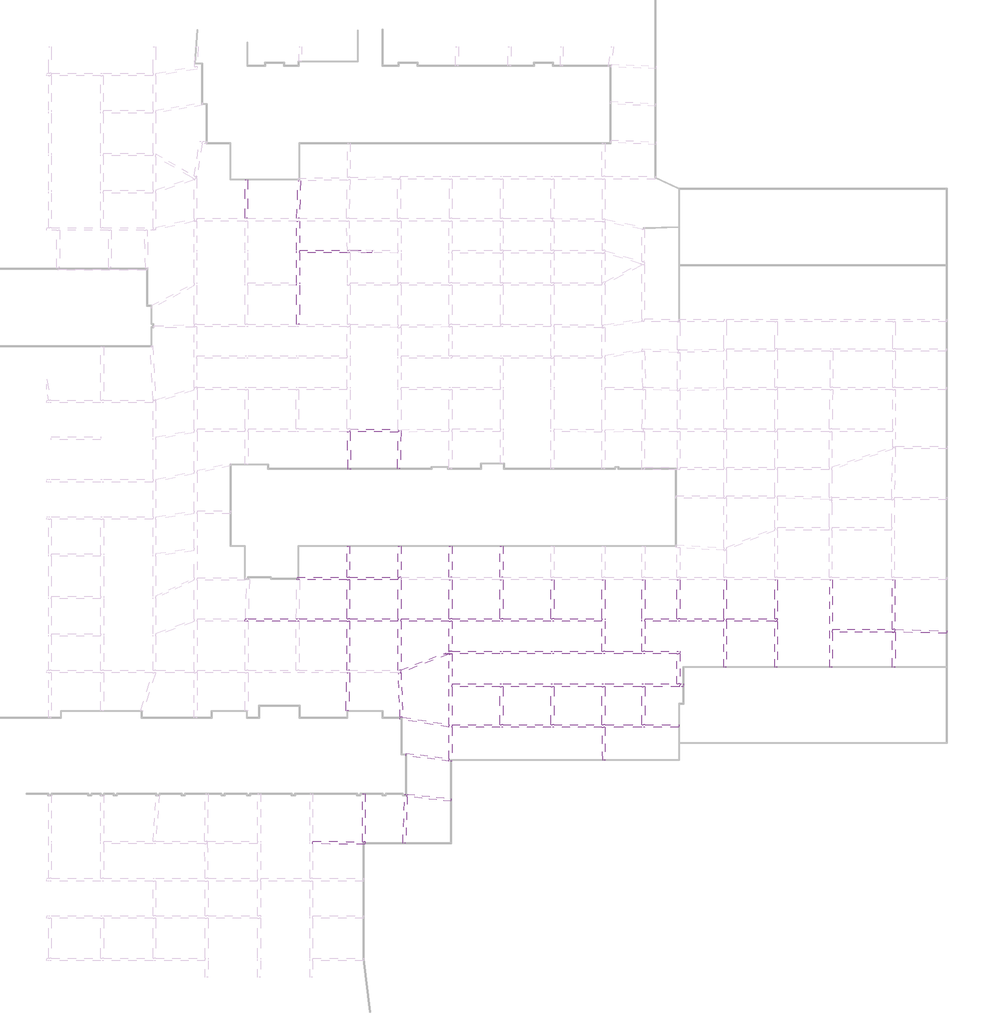
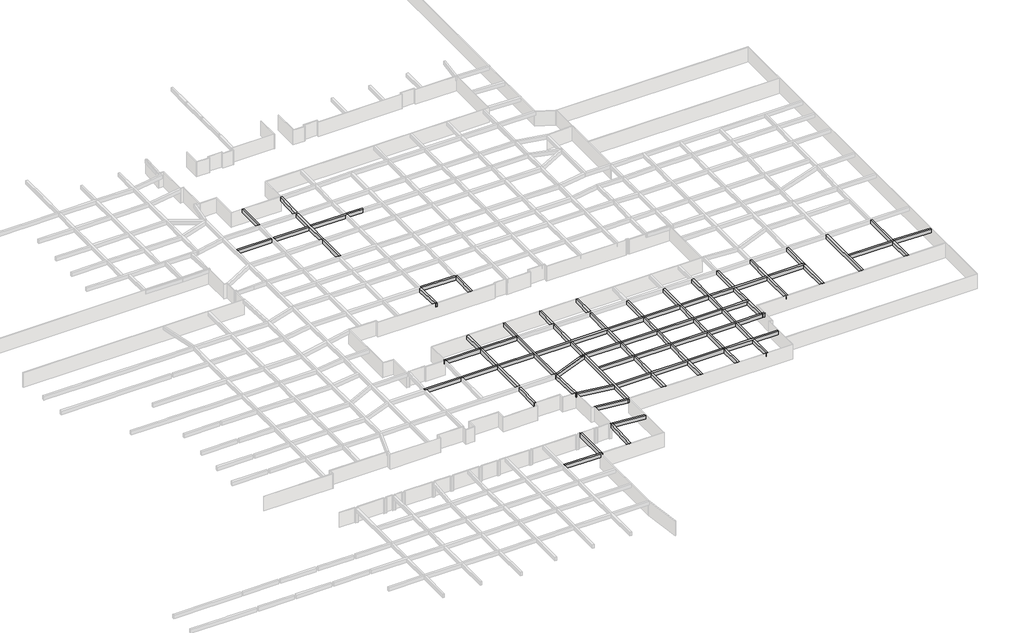
# One storey, part 13 of 20: 54 beams.
"""IFC4 building model written with IfcOpenShell, lengths in millimetres."""

from ifc_helpers import new_model, si_unit, frame, origin, place, context, project, spatial, polyline, outline, extrude, faceted_brep, element, save

model = new_model("IFC4")

# Units and contexts
model_context = context("Model", 3, world=origin())
ifc_project = project(units=[si_unit("LENGTHUNIT", "METRE", prefix="MILLI")], contexts=[model_context])

# Site, building, storey
site = spatial("IfcSite", under=ifc_project)
building = spatial("IfcBuilding", under=site)
storey = spatial("IfcBuildingStorey", under=building, Name="户型图", Elevation=0.0)

# Beams
placement = place(None, origin())
element("IfcBeam", 1, ObjectType="混凝土 - 矩形梁 : KL_beam", at=placement, inside=storey, context=model_context, shape_type="SweptSolid", body=[
    extrude(outline(polyline([(116499.0161386, 127439.0), (116899.0161386, 127439.0), (116899.0161386, 121489.0), (116499.0161386, 121489.0), (116499.0161386, 127439.0)])), frame((0.0, 0.0, 2500.0), z_axis=(0.0, 0.0, 1.0), x_axis=(1.0, 0.0, 0.0)), (0.0, 0.0, 1.0), 800.0),
])
element("IfcBeam", 2, ObjectType="混凝土 - 矩形梁 : KL_beam", at=placement, inside=storey, context=model_context, shape_type="SweptSolid", body=[
    extrude(outline(polyline([(124593.8863716, 127235.3718076), (124994.2683081, 127242.3605003), (124824.0062575, 121489.0), (124423.8311409, 121489.0), (124593.8863716, 127235.3718076)])), frame((0.0, 0.0, 2500.0), z_axis=(0.0, 0.0, 1.0), x_axis=(1.0, 0.0, 0.0)), (0.0, 0.0, 1.0), 800.0),
])
element("IfcBeam", 3, ObjectType="混凝土 - 矩形梁 : KL_beam", at=placement, inside=storey, context=model_context, shape_type="Brep", body=[
    faceted_brep([(134883.7348611, 26131.1937806, 3300.0), (134483.7348611, 26136.4805035, 3300.0), (126844.0, 26237.453407, 3300.0), (126844.0, 25837.4184717, 3300.0), (134878.4485999, 25731.2287128, 3300.0), (134878.4485999, 25731.2287128, 2500.0), (126844.0, 25837.4184717, 2500.0), (126844.0, 26237.453407, 2500.0), (134483.7348611, 26136.4805035, 2500.0), (134883.7348611, 26131.1937806, 2500.0)], [[[0, 1, 2, 3, 4]], [[5, 4, 3, 6]], [[6, 7, 8, 9, 5]], [[2, 1, 0, 9, 8, 7]], [[2, 7, 6, 3]], [[0, 4, 5, 9]]]),
])
element("IfcBeam", 4, ObjectType="混凝土 - 矩形梁 : KL_beam", at=placement, inside=storey, context=model_context, shape_type="Brep", body=[
    faceted_brep([(140350.0, 66590.0, 3300.0), (139950.0, 66590.0, 3300.0), (139950.0, 66190.0, 3300.0), (139950.0, 60290.0, 3300.0), (139950.0, 59890.0, 3300.0), (139950.0, 52365.0, 3300.0), (140350.0, 52365.0, 3300.0), (140350.0, 52453.6000936, 3300.0), (140350.0, 59890.0, 3300.0), (140350.0, 60290.0, 3300.0), (140350.0, 66190.0, 3300.0), (140350.0, 66590.0, 2500.0), (140350.0, 52365.0, 2500.0), (140350.0, 52453.6000936, 2500.0), (140350.0, 59890.0, 2500.0), (140350.0, 60290.0, 2500.0), (140350.0, 66190.0, 2500.0), (139950.0, 66590.0, 2500.0), (139950.0, 52365.0, 2500.0), (139950.0, 59890.0, 2500.0), (139950.0, 60290.0, 2500.0), (139950.0, 66190.0, 2500.0)], [[[0, 1, 2, 3, 4, 5, 6, 7, 8, 9, 10]], [[11, 0, 10, 9, 8, 7, 6, 12, 13, 14, 15, 16]], [[17, 11, 16, 15, 14, 13, 12, 18, 19, 20, 21]], [[1, 17, 21, 20, 19, 18, 5, 4, 3, 2]], [[6, 5, 18, 12]], [[1, 0, 11, 17]]]),
])
element("IfcBeam", 5, ObjectType="混凝土 - 矩形梁 : KL_beam", at=placement, inside=storey, context=model_context, shape_type="Brep", body=[
    faceted_brep([(124453.4605474, 66590.0, 3300.0), (124446.4785214, 66190.0, 3300.0), (124846.5394526, 66190.0, 3300.0), (132111.0, 66190.0, 3300.0), (132511.0, 66190.0, 3300.0), (139950.0, 66190.0, 3300.0), (139950.0, 66590.0, 3300.0), (132511.0, 66590.0, 3300.0), (132111.0, 66590.0, 3300.0), (124453.4605474, 66590.0, 2500.0), (139950.0, 66590.0, 2500.0), (132511.0, 66590.0, 2500.0), (132111.0, 66590.0, 2500.0), (124446.4785214, 66190.0, 2500.0), (139950.0, 66190.0, 2500.0), (132511.0, 66190.0, 2500.0), (132111.0, 66190.0, 2500.0), (124846.5394526, 66190.0, 2500.0)], [[[0, 1, 2, 3, 4, 5, 6, 7, 8]], [[9, 0, 8, 7, 6, 10, 11, 12]], [[13, 9, 12, 11, 10, 14, 15, 16, 17]], [[1, 13, 17, 16, 15, 14, 5, 4, 3, 2]], [[6, 5, 14, 10]], [[1, 0, 9, 13]]]),
])
element("IfcBeam", 6, ObjectType="混凝土 - 矩形梁 : KL_beam", at=placement, inside=storey, context=model_context, shape_type="Brep", body=[
    faceted_brep([(116550.0, 60290.0, 3300.0), (116550.0, 60254.832327, 3300.0), (116550.0, 59890.0, 3300.0), (116950.0, 59890.0, 3300.0), (124340.0498394, 59890.0, 3300.0), (124740.0498394, 59890.0, 3300.0), (132111.0, 59890.0, 3300.0), (132511.0, 59890.0, 3300.0), (139950.0, 59890.0, 3300.0), (139950.0, 60290.0, 3300.0), (132511.0, 60290.0, 3300.0), (132111.0, 60290.0, 3300.0), (124743.5545695, 60290.0, 3300.0), (124343.4936383, 60290.0, 3300.0), (116958.6197216, 60290.0, 3300.0), (116558.359171, 60290.0, 3300.0), (116550.0, 59890.0, 2500.0), (116950.0, 59890.0, 2500.0), (124340.0498394, 59890.0, 2500.0), (124740.0498394, 59890.0, 2500.0), (132111.0, 59890.0, 2500.0), (132511.0, 59890.0, 2500.0), (139950.0, 59890.0, 2500.0), (116550.0, 60254.832327, 2500.0), (116550.0, 60290.0, 2500.0), (116558.359171, 60290.0, 2500.0), (116958.6197216, 60290.0, 2500.0), (124343.4936383, 60290.0, 2500.0), (124743.5545695, 60290.0, 2500.0), (132111.0, 60290.0, 2500.0), (132511.0, 60290.0, 2500.0), (139950.0, 60290.0, 2500.0)], [[[0, 1, 2, 3, 4, 5, 6, 7, 8, 9, 10, 11, 12, 13, 14, 15]], [[2, 16, 17, 18, 19, 20, 21, 22, 8, 7, 6, 5, 4, 3]], [[16, 23, 24, 25, 26, 27, 28, 29, 30, 31, 22, 21, 20, 19, 18, 17]], [[24, 0, 15, 14, 13, 12, 11, 10, 9, 31, 30, 29, 28, 27, 26, 25]], [[9, 8, 22, 31]], [[2, 1, 0, 24, 23, 16]]]),
])
element("IfcBeam", 7, ObjectType="混凝土 - 矩形梁 : KL_beam", at=placement, inside=storey, context=model_context, shape_type="SweptSolid", body=[
    extrude(outline(polyline([(132111.0, 66190.0), (132511.0, 66190.0), (132511.0, 60290.0), (132111.0, 60290.0), (132111.0, 66190.0)])), frame((0.0, 0.0, 2500.0), z_axis=(0.0, 0.0, 1.0), x_axis=(1.0, 0.0, 0.0)), (0.0, 0.0, 1.0), 800.0),
])
element("IfcBeam", 8, ObjectType="混凝土 - 矩形梁 : KL_beam", at=placement, inside=storey, context=model_context, shape_type="SweptSolid", body=[
    extrude(outline(polyline([(132511.0, 52365.0), (132111.0, 52365.0), (132111.0, 59890.0), (132511.0, 59890.0), (132511.0, 52365.0)])), frame((0.0, 0.0, 2500.0), z_axis=(0.0, 0.0, 1.0), x_axis=(1.0, 0.0, 0.0)), (0.0, 0.0, 1.0), 800.0),
])
element("IfcBeam", 9, ObjectType="混凝土 - 矩形梁 : KL_beam", at=placement, inside=storey, context=model_context, shape_type="Brep", body=[
    faceted_brep([(140350.0, 60290.0, 3300.0), (140350.0, 59890.0, 3300.0), (147750.0, 59890.0, 3300.0), (148150.0, 59890.0, 3300.0), (155550.0, 59890.0, 3300.0), (155950.0, 59890.0, 3300.0), (163350.0, 59890.0, 3300.0), (163750.0, 59890.0, 3300.0), (171150.0, 59890.0, 3300.0), (171150.0, 60290.0, 3300.0), (163750.0, 60290.0, 3300.0), (163350.0, 60290.0, 3300.0), (155950.0, 60290.0, 3300.0), (155550.0, 60290.0, 3300.0), (148150.0, 60290.0, 3300.0), (147750.0, 60290.0, 3300.0), (140350.0, 59890.0, 2500.0), (147750.0, 59890.0, 2500.0), (148150.0, 59890.0, 2500.0), (155550.0, 59890.0, 2500.0), (155950.0, 59890.0, 2500.0), (163350.0, 59890.0, 2500.0), (163750.0, 59890.0, 2500.0), (171150.0, 59890.0, 2500.0), (140350.0, 60290.0, 2500.0), (147750.0, 60290.0, 2500.0), (148150.0, 60290.0, 2500.0), (155550.0, 60290.0, 2500.0), (155950.0, 60290.0, 2500.0), (163350.0, 60290.0, 2500.0), (163750.0, 60290.0, 2500.0), (171150.0, 60290.0, 2500.0)], [[[0, 1, 2, 3, 4, 5, 6, 7, 8, 9, 10, 11, 12, 13, 14, 15]], [[1, 16, 17, 18, 19, 20, 21, 22, 23, 8, 7, 6, 5, 4, 3, 2]], [[16, 24, 25, 26, 27, 28, 29, 30, 31, 23, 22, 21, 20, 19, 18, 17]], [[24, 0, 15, 14, 13, 12, 11, 10, 9, 31, 30, 29, 28, 27, 26, 25]], [[1, 0, 24, 16]], [[9, 8, 23, 31]]]),
])
element("IfcBeam", 10, ObjectType="混凝土 - 矩形梁 : KL_beam", at=placement, inside=storey, context=model_context, shape_type="Brep", body=[
    faceted_brep([(147913.7330836, 55290.0, 3300.0), (147750.0, 55228.6000936, 3300.0), (146847.066417, 54890.0, 3300.0), (147986.2669164, 54890.0, 3300.0), (148150.0, 54890.0, 3300.0), (155550.0, 54890.0, 3300.0), (155950.0, 54890.0, 3300.0), (163350.0, 54890.0, 3300.0), (163750.0, 54890.0, 3300.0), (171150.0, 54890.0, 3300.0), (171550.0, 54890.0, 3300.0), (177276.0, 54890.0, 3300.0), (177676.0, 54890.0, 3300.0), (182630.0, 54890.0, 3300.0), (183030.0, 54890.0, 3300.0), (183030.0, 55290.0, 3300.0), (182630.0, 55290.0, 3300.0), (177676.0, 55290.0, 3300.0), (177276.0, 55290.0, 3300.0), (171550.0, 55290.0, 3300.0), (171150.0, 55290.0, 3300.0), (163750.0, 55290.0, 3300.0), (163350.0, 55290.0, 3300.0), (155950.0, 55290.0, 3300.0), (155550.0, 55290.0, 3300.0), (148150.0, 55290.0, 3300.0), (146847.066417, 54890.0, 2500.0), (147986.2669164, 54890.0, 2500.0), (148150.0, 54890.0, 2500.0), (155550.0, 54890.0, 2500.0), (155950.0, 54890.0, 2500.0), (163350.0, 54890.0, 2500.0), (163750.0, 54890.0, 2500.0), (171150.0, 54890.0, 2500.0), (171550.0, 54890.0, 2500.0), (177276.0, 54890.0, 2500.0), (177676.0, 54890.0, 2500.0), (182630.0, 54890.0, 2500.0), (183030.0, 54890.0, 2500.0), (147750.0, 55228.6000936, 2500.0), (147913.7330836, 55290.0, 2500.0), (148150.0, 55290.0, 2500.0), (155550.0, 55290.0, 2500.0), (155950.0, 55290.0, 2500.0), (163350.0, 55290.0, 2500.0), (163750.0, 55290.0, 2500.0), (171150.0, 55290.0, 2500.0), (171550.0, 55290.0, 2500.0), (177276.0, 55290.0, 2500.0), (177676.0, 55290.0, 2500.0), (182630.0, 55290.0, 2500.0), (183030.0, 55290.0, 2500.0)], [[[0, 1, 2, 3, 4, 5, 6, 7, 8, 9, 10, 11, 12, 13, 14, 15, 16, 17, 18, 19, 20, 21, 22, 23, 24, 25]], [[2, 26, 27, 28, 29, 30, 31, 32, 33, 34, 35, 36, 37, 38, 14, 13, 12, 11, 10, 9, 8, 7, 6, 5, 4, 3]], [[26, 39, 40, 41, 42, 43, 44, 45, 46, 47, 48, 49, 50, 51, 38, 37, 36, 35, 34, 33, 32, 31, 30, 29, 28, 27]], [[40, 0, 25, 24, 23, 22, 21, 20, 19, 18, 17, 16, 15, 51, 50, 49, 48, 47, 46, 45, 44, 43, 42, 41]], [[2, 1, 0, 40, 39, 26]], [[15, 14, 38, 51]]]),
])
element("IfcBeam", 11, ObjectType="混凝土 - 矩形梁 : KL_beam", at=placement, inside=storey, context=model_context, shape_type="Brep", body=[
    faceted_brep([(183030.0, 49890.0, 3300.0), (183030.0, 50290.0, 3300.0), (182630.0, 50290.0, 3300.0), (177676.0, 50290.0, 3300.0), (177276.0, 50290.0, 3300.0), (171550.0, 50290.0, 3300.0), (171150.0, 50290.0, 3300.0), (163750.0, 50290.0, 3300.0), (163350.0, 50290.0, 3300.0), (155950.0, 50290.0, 3300.0), (155550.0, 50290.0, 3300.0), (148150.0, 50290.0, 3300.0), (148150.0, 49890.0, 3300.0), (155550.0, 49890.0, 3300.0), (155950.0, 49890.0, 3300.0), (163350.0, 49890.0, 3300.0), (163750.0, 49890.0, 3300.0), (171150.0, 49890.0, 3300.0), (171550.0, 49890.0, 3300.0), (177276.0, 49890.0, 3300.0), (177676.0, 49890.0, 3300.0), (183030.0, 49890.0, 2500.0), (148150.0, 49890.0, 2500.0), (155550.0, 49890.0, 2500.0), (155950.0, 49890.0, 2500.0), (163350.0, 49890.0, 2500.0), (163750.0, 49890.0, 2500.0), (171150.0, 49890.0, 2500.0), (171550.0, 49890.0, 2500.0), (177276.0, 49890.0, 2500.0), (177676.0, 49890.0, 2500.0), (183030.0, 50290.0, 2500.0), (148150.0, 50290.0, 2500.0), (155550.0, 50290.0, 2500.0), (155950.0, 50290.0, 2500.0), (163350.0, 50290.0, 2500.0), (163750.0, 50290.0, 2500.0), (171150.0, 50290.0, 2500.0), (171550.0, 50290.0, 2500.0), (177276.0, 50290.0, 2500.0), (177676.0, 50290.0, 2500.0), (182630.0, 50290.0, 2500.0)], [[[0, 1, 2, 3, 4, 5, 6, 7, 8, 9, 10, 11, 12, 13, 14, 15, 16, 17, 18, 19, 20]], [[21, 0, 20, 19, 18, 17, 16, 15, 14, 13, 12, 22, 23, 24, 25, 26, 27, 28, 29, 30]], [[31, 21, 30, 29, 28, 27, 26, 25, 24, 23, 22, 32, 33, 34, 35, 36, 37, 38, 39, 40, 41]], [[1, 31, 41, 40, 39, 38, 37, 36, 35, 34, 33, 32, 11, 10, 9, 8, 7, 6, 5, 4, 3, 2]], [[1, 0, 21, 31]], [[12, 11, 32, 22]]]),
])
element("IfcBeam", 12, ObjectType="混凝土 - 矩形梁 : KL_beam", at=placement, inside=storey, context=model_context, shape_type="Brep", body=[
    faceted_brep([(140350.0, 52453.6000936, 3300.0), (140350.0, 52365.0, 3300.0), (140350.0, 52026.3999064, 3300.0), (140355.7954074, 52028.5731842, 3300.0), (147750.0, 54801.3999064, 3300.0), (147986.2669164, 54890.0, 3300.0), (146847.066417, 54890.0, 3300.0), (140350.0, 52026.3999064, 2500.0), (140355.7954074, 52028.5731842, 2500.0), (147750.0, 54801.3999064, 2500.0), (147986.2669164, 54890.0, 2500.0), (140350.0, 52365.0, 2500.0), (140350.0, 52453.6000936, 2500.0), (146847.066417, 54890.0, 2500.0)], [[[0, 1, 2, 3, 4, 5, 6]], [[2, 7, 8, 9, 10, 5, 4, 3]], [[7, 11, 12, 13, 10, 9, 8]], [[12, 0, 6, 13]], [[7, 2, 1, 0, 12, 11]], [[6, 5, 10, 13]]]),
    faceted_brep([(139961.5516255, 51880.7317659, 2500.0), (139961.5516255, 51880.7317659, 3300.0), (139958.0768904, 51965.0, 3300.0), (139958.0768904, 51965.0, 2500.0), (140186.2669164, 51965.0, 3300.0), (140186.2669164, 51965.0, 2500.0)], [[[0, 1, 2, 3]], [[2, 4, 5, 3]], [[1, 4, 2]], [[1, 0, 5, 4]], [[5, 0, 3]]]),
])
element("IfcBeam", 13, ObjectType="混凝土 - 矩形梁 : KL_beam", at=placement, inside=storey, context=model_context, shape_type="SweptSolid", body=[
    extrude(outline(polyline([(148150.0, 55290.0), (147913.7330836, 55290.0), (147750.0, 55228.6000936), (147750.0, 59890.0), (148150.0, 59890.0), (148150.0, 55290.0)])), frame((0.0, 0.0, 2500.0), z_axis=(0.0, 0.0, 1.0), x_axis=(1.0, 0.0, 0.0)), (0.0, 0.0, 1.0), 800.0),
])
element("IfcBeam", 14, ObjectType="混凝土 - 矩形梁 : KL_beam", at=placement, inside=storey, context=model_context, shape_type="SweptSolid", body=[
    extrude(outline(polyline([(147750.0, 66190.0), (148150.0, 66190.0), (148150.0, 60290.0), (147750.0, 60290.0), (147750.0, 66190.0)])), frame((0.0, 0.0, 2500.0), z_axis=(0.0, 0.0, 1.0), x_axis=(1.0, 0.0, 0.0)), (0.0, 0.0, 1.0), 800.0),
])
element("IfcBeam", 15, ObjectType="混凝土 - 矩形梁 : KL_beam", at=placement, inside=storey, context=model_context, shape_type="SweptSolid", body=[
    extrude(outline(polyline([(155550.0, 66190.0), (155950.0, 66190.0), (155950.0, 60290.0), (155550.0, 60290.0), (155550.0, 66190.0)])), frame((0.0, 0.0, 2500.0), z_axis=(0.0, 0.0, 1.0), x_axis=(1.0, 0.0, 0.0)), (0.0, 0.0, 1.0), 800.0),
    extrude(outline(polyline([(155950.0, 50290.0), (155550.0, 50290.0), (155550.0, 54890.0), (155950.0, 54890.0), (155950.0, 50290.0)])), frame((0.0, 0.0, 2500.0), z_axis=(0.0, 0.0, 1.0), x_axis=(1.0, 0.0, 0.0)), (0.0, 0.0, 1.0), 800.0),
    extrude(outline(polyline([(155550.0, 59890.0), (155950.0, 59890.0), (155950.0, 55290.0), (155550.0, 55290.0), (155550.0, 59890.0)])), frame((0.0, 0.0, 2500.0), z_axis=(0.0, 0.0, 1.0), x_axis=(1.0, 0.0, 0.0)), (0.0, 0.0, 1.0), 800.0),
])
element("IfcBeam", 16, ObjectType="混凝土 - 矩形梁 : KL_beam", at=placement, inside=storey, context=model_context, shape_type="SweptSolid", body=[
    extrude(outline(polyline([(163750.0, 50290.0), (163350.0, 50290.0), (163350.0, 54890.0), (163750.0, 54890.0), (163750.0, 50290.0)])), frame((0.0, 0.0, 2500.0), z_axis=(0.0, 0.0, 1.0), x_axis=(1.0, 0.0, 0.0)), (0.0, 0.0, 1.0), 800.0),
    extrude(outline(polyline([(163350.0, 66190.0), (163750.0, 66190.0), (163750.0, 60290.0), (163350.0, 60290.0), (163350.0, 66190.0)])), frame((0.0, 0.0, 2500.0), z_axis=(0.0, 0.0, 1.0), x_axis=(1.0, 0.0, 0.0)), (0.0, 0.0, 1.0), 800.0),
    extrude(outline(polyline([(163350.0, 59890.0), (163750.0, 59890.0), (163750.0, 55290.0), (163350.0, 55290.0), (163350.0, 59890.0)])), frame((0.0, 0.0, 2500.0), z_axis=(0.0, 0.0, 1.0), x_axis=(1.0, 0.0, 0.0)), (0.0, 0.0, 1.0), 800.0),
])
element("IfcBeam", 17, ObjectType="混凝土 - 矩形梁 : KL_beam", at=placement, inside=storey, context=model_context, shape_type="Brep", body=[
    faceted_brep([(171550.0, 66190.0, 3300.0), (171150.0, 66190.0, 3300.0), (171150.0, 60290.0, 3300.0), (171150.0, 59890.0, 3300.0), (171150.0, 55290.0, 3300.0), (171550.0, 55290.0, 3300.0), (171550.0, 59890.0, 3300.0), (171550.0, 60290.0, 3300.0), (171150.0, 66190.0, 2500.0), (171150.0, 60290.0, 2500.0), (171150.0, 59890.0, 2500.0), (171150.0, 55290.0, 2500.0), (171550.0, 66190.0, 2500.0), (171550.0, 60290.0, 2500.0), (171550.0, 59890.0, 2500.0), (171550.0, 55290.0, 2500.0)], [[[0, 1, 2, 3, 4, 5, 6, 7]], [[1, 8, 9, 10, 11, 4, 3, 2]], [[8, 12, 13, 14, 15, 11, 10, 9]], [[12, 0, 7, 6, 5, 15, 14, 13]], [[1, 0, 12, 8]], [[5, 4, 11, 15]]]),
    faceted_brep([(171550.0, 50290.0, 3300.0), (171150.0, 50290.0, 3300.0), (171150.0, 50290.0, 2500.0), (171550.0, 50290.0, 2500.0), (171150.0, 54890.0, 3300.0), (171550.0, 54890.0, 3300.0), (171550.0, 54890.0, 2500.0), (171150.0, 54890.0, 2500.0)], [[[0, 1, 2, 3]], [[4, 5, 6, 7]], [[1, 0, 5, 4]], [[2, 1, 4, 7]], [[3, 2, 7, 6]], [[0, 3, 6, 5]]]),
])
element("IfcBeam", 18, ObjectType="混凝土 - 矩形梁 : KL_beam", at=placement, inside=storey, context=model_context, shape_type="Brep", body=[
    faceted_brep([(177276.0, 50290.0, 3300.0), (177676.0, 50290.0, 3300.0), (177676.0, 54890.0, 3300.0), (177276.0, 54890.0, 3300.0), (177676.0, 50290.0, 2500.0), (177676.0, 54890.0, 2500.0), (177276.0, 50290.0, 2500.0), (177276.0, 54890.0, 2500.0)], [[[0, 1, 2, 3]], [[1, 4, 5, 2]], [[4, 6, 7, 5]], [[6, 0, 3, 7]], [[1, 0, 6, 4]], [[3, 2, 5, 7]]]),
    faceted_brep([(177276.0, 66190.0, 3300.0), (177676.0, 66190.0, 3300.0), (177676.0, 66190.0, 2500.0), (177276.0, 66190.0, 2500.0), (177676.0, 55290.0, 3300.0), (177276.0, 55290.0, 3300.0), (177276.0, 55290.0, 2500.0), (177676.0, 55290.0, 2500.0), (177276.0, 60290.0, 3300.0), (177276.0, 59890.0, 3300.0), (177676.0, 59890.0, 3300.0), (177676.0, 60290.0, 3300.0), (177676.0, 59890.0, 2500.0), (177676.0, 60290.0, 2500.0), (177276.0, 59890.0, 2500.0), (177276.0, 60290.0, 2500.0)], [[[0, 1, 2, 3]], [[4, 5, 6, 7]], [[1, 0, 8, 9, 5, 4, 10, 11]], [[2, 1, 11, 10, 4, 7, 12, 13]], [[3, 2, 13, 12, 7, 6, 14, 15]], [[0, 3, 15, 14, 6, 5, 9, 8]]]),
])
element("IfcBeam", 19, ObjectType="混凝土 - 矩形梁 : KL_beam", at=placement, inside=storey, context=model_context, shape_type="Brep", body=[
    faceted_brep([(171550.0, 60290.0, 3300.0), (171550.0, 59890.0, 3300.0), (177276.0, 59890.0, 3300.0), (177276.0, 60290.0, 3300.0), (171550.0, 59890.0, 2500.0), (177276.0, 59890.0, 2500.0), (171550.0, 60290.0, 2500.0), (177276.0, 60290.0, 2500.0)], [[[0, 1, 2, 3]], [[1, 4, 5, 2]], [[4, 6, 7, 5]], [[6, 0, 3, 7]], [[1, 0, 6, 4]], [[3, 2, 5, 7]]]),
    faceted_brep([(177676.0, 59890.0, 3300.0), (177676.0, 60290.0, 3300.0), (177676.0, 60290.0, 2500.0), (177676.0, 59890.0, 2500.0), (182630.0, 59890.0, 3300.0), (183030.0, 59890.0, 3300.0), (189762.0, 59890.0, 3300.0), (189762.0, 60290.0, 3300.0), (183030.0, 60290.0, 3300.0), (182630.0, 60290.0, 3300.0), (182630.0, 59890.0, 2500.0), (183030.0, 59890.0, 2500.0), (189762.0, 59890.0, 2500.0), (182630.0, 60290.0, 2500.0), (183030.0, 60290.0, 2500.0), (189762.0, 60290.0, 2500.0)], [[[0, 1, 2, 3]], [[1, 0, 4, 5, 6, 7, 8, 9]], [[0, 3, 10, 11, 12, 6, 5, 4]], [[3, 2, 13, 14, 15, 12, 11, 10]], [[2, 1, 9, 8, 7, 15, 14, 13]], [[7, 6, 12, 15]]]),
])
element("IfcBeam", 20, ObjectType="混凝土 - 矩形梁 : KL_beam", at=placement, inside=storey, context=model_context, shape_type="SweptSolid", body=[
    extrude(outline(polyline([(182630.0, 66190.0), (183030.0, 66190.0), (183030.0, 60290.0), (182630.0, 60290.0), (182630.0, 66190.0)])), frame((0.0, 0.0, 2500.0), z_axis=(0.0, 0.0, 1.0), x_axis=(1.0, 0.0, 0.0)), (0.0, 0.0, 1.0), 800.0),
    extrude(outline(polyline([(183030.0, 55290.0), (182630.0, 55290.0), (182630.0, 59890.0), (183030.0, 59890.0), (183030.0, 55290.0)])), frame((0.0, 0.0, 2500.0), z_axis=(0.0, 0.0, 1.0), x_axis=(1.0, 0.0, 0.0)), (0.0, 0.0, 1.0), 800.0),
])
element("IfcBeam", 21, ObjectType="混凝土 - 矩形梁 : KL_beam", at=placement, inside=storey, context=model_context, shape_type="SweptSolid", body=[
    extrude(outline(polyline([(182630.0, 54890.0), (183030.0, 54890.0), (183030.0, 50290.0), (182630.0, 50290.0), (182630.0, 54890.0)])), frame((0.0, 0.0, 2500.0), z_axis=(0.0, 0.0, 1.0), x_axis=(1.0, 0.0, 0.0)), (0.0, 0.0, 1.0), 800.0),
])
element("IfcBeam", 22, ObjectType="混凝土 - 矩形梁 : KL_beam", at=placement, inside=storey, context=model_context, shape_type="SweptSolid", body=[
    extrude(outline(polyline([(183590.0, 50290.0), (183590.0, 49890.0), (183030.0, 49890.0), (183030.0, 50290.0), (183590.0, 50290.0)])), frame((0.0, 0.0, 2500.0), z_axis=(0.0, 0.0, 1.0), x_axis=(1.0, 0.0, 0.0)), (0.0, 0.0, 1.0), 800.0),
])
element("IfcBeam", 23, ObjectType="混凝土 - 矩形梁 : KL_beam", at=placement, inside=storey, context=model_context, shape_type="Brep", body=[
    faceted_brep([(197950.0, 59890.0, 3300.0), (197950.0, 60290.0, 3300.0), (197562.0, 60290.0, 3300.0), (190162.0, 60290.0, 3300.0), (190162.0, 59890.0, 3300.0), (197550.0, 59890.0, 3300.0), (197950.0, 59890.0, 2500.0), (190162.0, 59890.0, 2500.0), (197550.0, 59890.0, 2500.0), (197950.0, 60290.0, 2500.0), (190162.0, 60290.0, 2500.0), (197562.0, 60290.0, 2500.0)], [[[0, 1, 2, 3, 4, 5]], [[6, 0, 5, 4, 7, 8]], [[9, 6, 8, 7, 10, 11]], [[1, 9, 11, 10, 3, 2]], [[1, 0, 6, 9]], [[4, 3, 10, 7]]]),
])
element("IfcBeam", 24, ObjectType="混凝土 - 矩形梁 : KL_beam", at=placement, inside=storey, context=model_context, shape_type="Brep", body=[
    faceted_brep([(197550.0, 52865.0, 3300.0), (197550.0, 52865.0, 2500.0), (197950.0, 52865.0, 2500.0), (197950.0, 52865.0, 3300.0), (197950.0, 59790.0, 3300.0), (197950.0, 59890.0, 3300.0), (197550.0, 59890.0, 3300.0), (197950.0, 59790.0, 2500.0), (197950.0, 59890.0, 2500.0), (197550.0, 59890.0, 2500.0)], [[[0, 1, 2, 3]], [[0, 3, 4, 5, 6]], [[3, 2, 7, 8, 5, 4]], [[2, 1, 9, 8, 7]], [[1, 0, 6, 9]], [[6, 5, 8, 9]]]),
])
element("IfcBeam", 25, ObjectType="混凝土 - 矩形梁 : KL_beam", at=placement, inside=storey, context=model_context, shape_type="Brep", body=[
    faceted_brep([(190162.0, 52865.0, 3300.0), (189762.0, 52865.0, 3300.0), (189762.0, 52865.0, 2500.0), (190162.0, 52865.0, 2500.0), (190162.0, 59890.0, 3300.0), (190162.0, 60290.0, 3300.0), (190162.0, 66190.0, 3300.0), (189762.0, 66190.0, 3300.0), (189762.0, 60290.0, 3300.0), (189762.0, 59890.0, 3300.0), (189762.0, 66190.0, 2500.0), (189762.0, 60290.0, 2500.0), (189762.0, 59890.0, 2500.0), (190162.0, 66190.0, 2500.0), (190162.0, 60290.0, 2500.0), (190162.0, 59890.0, 2500.0)], [[[0, 1, 2, 3]], [[1, 0, 4, 5, 6, 7, 8, 9]], [[2, 1, 9, 8, 7, 10, 11, 12]], [[3, 2, 12, 11, 10, 13, 14, 15]], [[0, 3, 15, 14, 13, 6, 5, 4]], [[7, 6, 13, 10]]]),
])
element("IfcBeam", 26, ObjectType="混凝土 - 矩形梁 : KL_beam", at=placement, inside=storey, context=model_context, shape_type="Brep", body=[
    faceted_brep([(197962.0, 59790.0, 2500.0), (197962.0, 59790.0, 3300.0), (197950.0, 59790.0, 3300.0), (197950.0, 59790.0, 2500.0), (197962.0, 66190.0, 3300.0), (197562.0, 66190.0, 3300.0), (197562.0, 60290.0, 3300.0), (197950.0, 60290.0, 3300.0), (197950.0, 59890.0, 3300.0), (197962.0, 66190.0, 2500.0), (197950.0, 59890.0, 2500.0), (197950.0, 60290.0, 2500.0), (197562.0, 60290.0, 2500.0), (197562.0, 66190.0, 2500.0)], [[[0, 1, 2, 3]], [[1, 4, 5, 6, 7, 8, 2]], [[9, 0, 3, 10, 11, 12, 13]], [[1, 0, 9, 4]], [[5, 4, 9, 13]], [[11, 7, 6, 12]], [[7, 11, 10, 3, 2, 8]], [[5, 13, 12, 6]]]),
])
element("IfcBeam", 27, ObjectType="混凝土 - 矩形梁 : KL_beam", at=placement, inside=storey, context=model_context, shape_type="Brep", body=[
    faceted_brep([(206362.0, 52865.0, 3300.0), (205962.0, 52865.0, 3300.0), (205962.0, 52865.0, 2500.0), (206362.0, 52865.0, 2500.0), (206362.0, 58225.0, 3300.0), (206362.0, 58625.0, 3300.0), (206362.0, 66190.0, 3300.0), (205962.0, 66190.0, 3300.0), (205962.0, 66190.0, 2500.0), (206362.0, 66190.0, 2500.0), (206362.0, 58625.0, 2500.0), (206362.0, 58225.0, 2500.0)], [[[0, 1, 2, 3]], [[1, 0, 4, 5, 6, 7]], [[2, 1, 7, 8]], [[3, 2, 8, 9, 10, 11]], [[0, 3, 11, 10, 9, 6, 5, 4]], [[7, 6, 9, 8]]]),
])
element("IfcBeam", 28, ObjectType="混凝土 - 矩形梁 : KL_beam", at=placement, inside=storey, context=model_context, shape_type="Brep", body=[
    faceted_brep([(215938.0, 58225.0, 3300.0), (215938.0, 58619.7587752, 3300.0), (215938.0, 58625.0, 3300.0), (215538.0, 58625.0, 3300.0), (206362.0, 58625.0, 3300.0), (206362.0, 58225.0, 3300.0), (215587.3766771, 58225.0, 3300.0), (215735.3445936, 58225.0, 3300.0), (215938.0, 58225.0, 2500.0), (206362.0, 58225.0, 2500.0), (215587.3766771, 58225.0, 2500.0), (215735.3445936, 58225.0, 2500.0), (215938.0, 58625.0, 2500.0), (215938.0, 58619.7587752, 2500.0), (206362.0, 58625.0, 2500.0), (215538.0, 58625.0, 2500.0)], [[[0, 1, 2, 3, 4, 5, 6, 7]], [[8, 0, 7, 6, 5, 9, 10, 11]], [[12, 13, 8, 11, 10, 9, 14, 15]], [[2, 12, 15, 14, 4, 3]], [[5, 4, 14, 9]], [[2, 1, 0, 8, 13, 12]]]),
])
element("IfcBeam", 29, ObjectType="混凝土 - 矩形梁 : KL_beam", at=placement, inside=storey, context=model_context, shape_type="SweptSolid", body=[
    extrude(outline(polyline([(215938.0, 58625.0), (215538.0, 58625.0), (215538.0, 66190.0), (215938.0, 66190.0), (215938.0, 58625.0)])), frame((0.0, 0.0, 2500.0), z_axis=(0.0, 0.0, 1.0), x_axis=(1.0, 0.0, 0.0)), (0.0, 0.0, 1.0), 800.0),
])
element("IfcBeam", 30, ObjectType="混凝土 - 矩形梁 : KL_beam", at=placement, inside=storey, context=model_context, shape_type="Brep", body=[
    faceted_brep([(223902.8713364, 58408.2217851, 3300.0), (223892.251583, 58008.3627839, 3300.0), (223892.251583, 58008.3627839, 2500.0), (223902.8713364, 58408.2217851, 2500.0), (215938.0, 58619.7587752, 3300.0), (215938.0, 58225.0, 3300.0), (215735.3445936, 58225.0, 3300.0), (215987.3766771, 58218.3063441, 3300.0), (215735.3445936, 58225.0, 2500.0), (215987.3766771, 58218.3063441, 2500.0), (215938.0, 58225.0, 2500.0), (215938.0, 58619.7587752, 2500.0)], [[[0, 1, 2, 3]], [[1, 0, 4, 5, 6, 7]], [[2, 1, 7, 6, 8, 9]], [[3, 2, 9, 8, 10, 11]], [[0, 3, 11, 4]], [[5, 10, 8, 6]], [[10, 5, 4, 11]]]),
])
element("IfcBeam", 31, ObjectType="混凝土 - 矩形梁 : KL_beam", at=placement, inside=storey, context=model_context, shape_type="SweptSolid", body=[
    extrude(outline(polyline([(215987.3766771, 52865.0), (215587.3766771, 52865.0), (215587.3766771, 58225.0), (215735.3445936, 58225.0), (215987.3766771, 58218.3063441), (215987.3766771, 52865.0)])), frame((0.0, 0.0, 2500.0), z_axis=(0.0, 0.0, 1.0), x_axis=(1.0, 0.0, 0.0)), (0.0, 0.0, 1.0), 800.0),
])
element("IfcBeam", 32, ObjectType="混凝土 - 矩形梁 : KL_beam", at=placement, inside=storey, context=model_context, shape_type="Brep", body=[
    faceted_brep([(182924.9999998, 44040.0, 3300.0), (182924.9999998, 43640.0, 3300.0), (182924.9999998, 43640.0, 2500.0), (182924.9999998, 44040.0, 2500.0), (177676.0, 44040.0, 3300.0), (177276.0, 44040.0, 3300.0), (171550.0, 44040.0, 3300.0), (171150.0, 44040.0, 3300.0), (163750.0, 44040.0, 3300.0), (163350.0, 44040.0, 3300.0), (155950.0, 44040.0, 3300.0), (155550.0, 44040.0, 3300.0), (148150.0, 44040.0, 3300.0), (148150.0, 43640.0, 3300.0), (155550.0, 43640.0, 3300.0), (155950.0, 43640.0, 3300.0), (163350.0, 43640.0, 3300.0), (163750.0, 43640.0, 3300.0), (171153.4605474, 43640.0, 3300.0), (171553.5214786, 43640.0, 3300.0), (177276.0, 43640.0, 3300.0), (177676.0, 43640.0, 3300.0), (148150.0, 43640.0, 2500.0), (155550.0, 43640.0, 2500.0), (155950.0, 43640.0, 2500.0), (163350.0, 43640.0, 2500.0), (163750.0, 43640.0, 2500.0), (171153.4605474, 43640.0, 2500.0), (171553.5214786, 43640.0, 2500.0), (177276.0, 43640.0, 2500.0), (177676.0, 43640.0, 2500.0), (148150.0, 44040.0, 2500.0), (155550.0, 44040.0, 2500.0), (155950.0, 44040.0, 2500.0), (163350.0, 44040.0, 2500.0), (163750.0, 44040.0, 2500.0), (171150.0, 44040.0, 2500.0), (171550.0, 44040.0, 2500.0), (177276.0, 44040.0, 2500.0), (177676.0, 44040.0, 2500.0)], [[[0, 1, 2, 3]], [[1, 0, 4, 5, 6, 7, 8, 9, 10, 11, 12, 13, 14, 15, 16, 17, 18, 19, 20, 21]], [[2, 1, 21, 20, 19, 18, 17, 16, 15, 14, 13, 22, 23, 24, 25, 26, 27, 28, 29, 30]], [[3, 2, 30, 29, 28, 27, 26, 25, 24, 23, 22, 31, 32, 33, 34, 35, 36, 37, 38, 39]], [[0, 3, 39, 38, 37, 36, 35, 34, 33, 32, 31, 12, 11, 10, 9, 8, 7, 6, 5, 4]], [[13, 12, 31, 22]]]),
])
element("IfcBeam", 33, ObjectType="混凝土 - 矩形梁 : KL_beam", at=placement, inside=storey, context=model_context, shape_type="SweptSolid", body=[
    extrude(outline(polyline([(163750.0, 38640.0), (163350.0, 38640.0), (163350.0, 43640.0), (163750.0, 43640.0), (163750.0, 38640.0)])), frame((0.0, 0.0, 2500.0), z_axis=(0.0, 0.0, 1.0), x_axis=(1.0, 0.0, 0.0)), (0.0, 0.0, 1.0), 800.0),
    extrude(outline(polyline([(163350.0, 49890.0), (163750.0, 49890.0), (163750.0, 44040.0), (163350.0, 44040.0), (163350.0, 49890.0)])), frame((0.0, 0.0, 2500.0), z_axis=(0.0, 0.0, 1.0), x_axis=(1.0, 0.0, 0.0)), (0.0, 0.0, 1.0), 800.0),
])
element("IfcBeam", 34, ObjectType="混凝土 - 矩形梁 : KL_beam", at=placement, inside=storey, context=model_context, shape_type="SweptSolid", body=[
    extrude(outline(polyline([(171150.0, 49890.0), (171550.0, 49890.0), (171550.0, 44040.0), (171150.0, 44040.0), (171150.0, 49890.0)])), frame((0.0, 0.0, 2500.0), z_axis=(0.0, 0.0, 1.0), x_axis=(1.0, 0.0, 0.0)), (0.0, 0.0, 1.0), 800.0),
])
element("IfcBeam", 35, ObjectType="混凝土 - 矩形梁 : KL_beam", at=placement, inside=storey, context=model_context, shape_type="SweptSolid", body=[
    extrude(outline(polyline([(171640.7289646, 38643.8864739), (171240.7898865, 38636.9055113), (171153.4605474, 43640.0), (171553.5214786, 43640.0), (171640.7289646, 38643.8864739)])), frame((0.0, 0.0, 2500.0), z_axis=(0.0, 0.0, 1.0), x_axis=(1.0, 0.0, 0.0)), (0.0, 0.0, 1.0), 800.0),
])
element("IfcBeam", 36, ObjectType="混凝土 - 矩形梁 : KL_beam", at=placement, inside=storey, context=model_context, shape_type="SweptSolid", body=[
    extrude(outline(polyline([(177676.0, 38640.0), (177276.0, 38640.0), (177276.0, 43640.0), (177676.0, 43640.0), (177676.0, 38640.0)])), frame((0.0, 0.0, 2500.0), z_axis=(0.0, 0.0, 1.0), x_axis=(1.0, 0.0, 0.0)), (0.0, 0.0, 1.0), 800.0),
    extrude(outline(polyline([(177276.0, 49890.0), (177676.0, 49890.0), (177676.0, 44040.0), (177276.0, 44040.0), (177276.0, 49890.0)])), frame((0.0, 0.0, 2500.0), z_axis=(0.0, 0.0, 1.0), x_axis=(1.0, 0.0, 0.0)), (0.0, 0.0, 1.0), 800.0),
])
element("IfcBeam", 37, ObjectType="混凝土 - 矩形梁 : KL_beam", at=placement, inside=storey, context=model_context, shape_type="Brep", body=[
    faceted_brep([(148150.0, 38463.8482621, 3300.0), (148150.0, 43640.0, 3300.0), (148150.0, 44040.0, 3300.0), (148150.0, 49890.0, 3300.0), (148150.0, 50290.0, 3300.0), (148150.0, 54890.0, 3300.0), (147986.2669164, 54890.0, 3300.0), (147750.0, 54801.3999064, 3300.0), (147750.0, 44074.359987, 3300.0), (147750.0, 43669.3224005, 3300.0), (147750.0, 38867.0769535, 3300.0), (147750.0, 38463.8482621, 3300.0), (147750.0, 54801.3999064, 2500.0), (147750.0, 44074.359987, 2500.0), (147750.0, 43669.3224005, 2500.0), (147750.0, 38867.0769535, 2500.0), (147750.0, 38463.8482621, 2500.0), (148150.0, 54890.0, 2500.0), (148150.0, 50290.0, 2500.0), (148150.0, 49890.0, 2500.0), (148150.0, 44040.0, 2500.0), (148150.0, 43640.0, 2500.0), (148150.0, 38463.8482621, 2500.0), (147986.2669164, 54890.0, 2500.0)], [[[0, 1, 2, 3, 4, 5, 6, 7, 8, 9, 10, 11]], [[11, 10, 9, 8, 7, 12, 13, 14, 15, 16]], [[17, 18, 19, 20, 21, 22, 16, 15, 14, 13, 12, 23]], [[5, 4, 3, 2, 1, 0, 22, 21, 20, 19, 18, 17]], [[5, 17, 23, 6]], [[7, 6, 23, 12]], [[0, 11, 16, 22]]]),
])
element("IfcBeam", 38, ObjectType="混凝土 - 矩形梁 : KL_beam", at=placement, inside=storey, context=model_context, shape_type="Brep", body=[
    faceted_brep([(140234.1014129, 45270.9359011, 3300.0), (140250.9131873, 44863.2217798, 3300.0), (147750.0, 43669.3224005, 3300.0), (147750.0, 44074.359987, 3300.0), (140637.0868127, 45206.7782202, 3300.0), (140250.9131873, 44863.2217798, 2500.0), (147750.0, 43669.3224005, 2500.0), (140234.1014129, 45270.9359011, 2500.0), (140637.0868127, 45206.7782202, 2500.0), (147750.0, 44074.359987, 2500.0)], [[[0, 1, 2, 3, 4]], [[1, 5, 6, 2]], [[5, 7, 8, 9, 6]], [[7, 0, 4, 3, 9, 8]], [[3, 2, 6, 9]], [[1, 0, 7, 5]]]),
])
element("IfcBeam", 39, ObjectType="混凝土 - 矩形梁 : KL_beam", at=placement, inside=storey, context=model_context, shape_type="SweptSolid", body=[
    extrude(outline(polyline([(140186.2669164, 51965.0), (140350.0, 51965.0), (140350.0, 52026.3999064), (140355.7954074, 52028.5731842), (140637.0868127, 45206.7782202), (140234.1014129, 45270.9359011), (139961.5516255, 51880.7317659), (140186.2669164, 51965.0)])), frame((0.0, 0.0, 2500.0), z_axis=(0.0, 0.0, 1.0), x_axis=(1.0, 0.0, 0.0)), (0.0, 0.0, 1.0), 800.0),
])
element("IfcBeam", 40, ObjectType="混凝土 - 矩形梁 : KL_beam", at=placement, inside=storey, context=model_context, shape_type="SweptSolid", body=[
    extrude(outline(polyline([(132347.9292728, 46152.6805044), (131948.0764532, 46163.5305143), (132105.4993808, 51965.0), (132505.6466155, 51965.0), (132347.9292728, 46152.6805044)])), frame((0.0, 0.0, 2500.0), z_axis=(0.0, 0.0, 1.0), x_axis=(1.0, 0.0, 0.0)), (0.0, 0.0, 1.0), 800.0),
])
element("IfcBeam", 41, ObjectType="混凝土 - 矩形梁 : KL_beam", at=placement, inside=storey, context=model_context, shape_type="SweptSolid", body=[
    extrude(outline(polyline([(141107.3333896, 39309.5463365), (141157.8508421, 39706.3434975), (147750.0, 38867.0769535), (147750.0, 38463.8482621), (141107.3333896, 39309.5463365)])), frame((0.0, 0.0, 2500.0), z_axis=(0.0, 0.0, 1.0), x_axis=(1.0, 0.0, 0.0)), (0.0, 0.0, 1.0), 800.0),
])
element("IfcBeam", 42, ObjectType="混凝土 - 矩形梁 : KL_beam", at=placement, inside=storey, context=model_context, shape_type="Brep", body=[
    faceted_brep([(141076.3490671, 25928.0578427, 3300.0), (140676.5927363, 25942.0176414, 3300.0), (140676.5927363, 25942.0176414, 2500.0), (141076.3490671, 25928.0578427, 2500.0), (141324.5525977, 33035.6770103, 3300.0), (141338.5464848, 33436.4095053, 3300.0), (140938.790154, 33450.369304, 3300.0), (140938.790154, 33450.369304, 2500.0), (141338.5464848, 33436.4095053, 2500.0), (141324.5525977, 33035.6770103, 2500.0)], [[[0, 1, 2, 3]], [[1, 0, 4, 5, 6]], [[2, 1, 6, 7]], [[3, 2, 7, 8, 9]], [[0, 3, 9, 8, 5, 4]], [[5, 8, 7, 6]]]),
])
element("IfcBeam", 43, ObjectType="混凝土 - 矩形梁 : KL_beam", at=placement, inside=storey, context=model_context, shape_type="SweptSolid", body=[
    extrude(outline(polyline([(148060.4627033, 32729.9076416), (148018.651318, 32332.0988835), (141324.5525977, 33035.6770103), (141338.5464848, 33436.4095053), (148060.4627033, 32729.9076416)])), frame((0.0, 0.0, 2500.0), z_axis=(0.0, 0.0, 1.0), x_axis=(1.0, 0.0, 0.0)), (0.0, 0.0, 1.0), 800.0),
])
element("IfcBeam", 44, ObjectType="混凝土 - 矩形梁 : KL_beam", at=placement, inside=storey, context=model_context, shape_type="Brep", body=[
    faceted_brep([(134883.7348611, 33506.9098372, 3300.0), (134883.7348611, 33506.9098372, 2500.0), (134483.7348611, 33506.9098372, 2500.0), (134483.7348611, 33506.9098372, 3300.0), (134878.4485999, 25731.2287128, 3300.0), (134883.7348611, 25731.1588453, 3300.0), (134883.7348611, 26131.1937806, 3300.0), (134483.7348611, 26136.4805035, 2500.0), (134483.7348611, 26136.4805035, 3300.0), (134883.7348611, 25731.1588453, 2500.0), (134878.4485999, 25731.2287128, 2500.0), (134883.7348611, 26131.1937806, 2500.0)], [[[0, 1, 2, 3]], [[4, 5, 6]], [[3, 2, 7, 8]], [[9, 10, 11]], [[1, 0, 6, 5, 9, 11]], [[9, 5, 4, 10]], [[11, 6, 8, 7]], [[6, 11, 10, 4]], [[0, 3, 8, 6]], [[2, 1, 11, 7]]]),
])
element("IfcBeam", 45, ObjectType="混凝土 - 矩形梁 : KL_beam", at=placement, inside=storey, context=model_context, shape_type="SweptSolid", body=[
    extrude(outline(polyline([(155950.0, 38640.0), (155550.0, 38640.0), (155550.0, 43640.0), (155950.0, 43640.0), (155950.0, 38640.0)])), frame((0.0, 0.0, 2500.0), z_axis=(0.0, 0.0, 1.0), x_axis=(1.0, 0.0, 0.0)), (0.0, 0.0, 1.0), 800.0),
    extrude(outline(polyline([(155550.0, 49890.0), (155950.0, 49890.0), (155950.0, 44040.0), (155550.0, 44040.0), (155550.0, 49890.0)])), frame((0.0, 0.0, 2500.0), z_axis=(0.0, 0.0, 1.0), x_axis=(1.0, 0.0, 0.0)), (0.0, 0.0, 1.0), 800.0),
])
element("IfcBeam", 46, ObjectType="混凝土 - 矩形梁 : KL_beam", at=placement, inside=storey, context=model_context, shape_type="Brep", body=[
    faceted_brep([(132700.4140676, 83156.9729496, 3300.0), (132300.5424408, 83146.8397338, 3300.0), (132300.5424408, 83146.8397338, 2500.0), (132700.4140676, 83156.9729496, 2500.0), (132555.1995248, 88887.352801, 3300.0), (132555.1324416, 88890.0, 3300.0), (132155.0040273, 88890.0, 3300.0), (132155.0040273, 88890.0, 2500.0), (132555.1324416, 88890.0, 2500.0), (132555.1995248, 88887.352801, 2500.0)], [[[0, 1, 2, 3]], [[1, 0, 4, 5, 6]], [[2, 1, 6, 7]], [[3, 2, 7, 8, 9]], [[0, 3, 9, 8, 5, 4]], [[6, 5, 8, 7]]]),
])
element("IfcBeam", 47, ObjectType="混凝土 - 矩形梁 : KL_beam", at=placement, inside=storey, context=model_context, shape_type="Brep", body=[
    faceted_brep([(140249.2614841, 83216.9489182, 3300.0), (139849.3224061, 83223.9298808, 3300.0), (139849.3224061, 83223.9298808, 2500.0), (140249.2614841, 83216.9489182, 2500.0), (140346.5831577, 88792.503861, 3300.0), (140350.0, 88988.2546264, 3300.0), (139950.0, 88991.7453736, 3300.0), (139946.523769, 88792.5922337, 3300.0), (139950.0, 88991.7453736, 2500.0), (139946.523769, 88792.5922337, 2500.0), (140350.0, 88988.2546264, 2500.0), (140346.5831577, 88792.503861, 2500.0)], [[[0, 1, 2, 3]], [[1, 0, 4, 5, 6, 7]], [[2, 1, 7, 6, 8, 9]], [[3, 2, 9, 8, 10, 11]], [[0, 3, 11, 10, 5, 4]], [[5, 10, 8, 6]]]),
])
element("IfcBeam", 48, ObjectType="混凝土 - 矩形梁 : KL_beam", at=placement, inside=storey, context=model_context, shape_type="Brep", body=[
    faceted_brep([(132550.0, 89092.5337107, 3300.0), (132555.1324416, 88890.0, 3300.0), (132555.1995248, 88887.352801, 3300.0), (139946.523769, 88792.5922337, 3300.0), (139950.0, 88991.7453736, 3300.0), (139950.0, 89192.5805384, 3300.0), (132550.0, 89287.4523333, 3300.0), (132555.1995248, 88887.352801, 2500.0), (139946.523769, 88792.5922337, 2500.0), (132555.1324416, 88890.0, 2500.0), (132550.0, 89092.5337107, 2500.0), (132550.0, 89287.4523333, 2500.0), (139950.0, 89192.5805384, 2500.0), (139950.0, 88991.7453736, 2500.0)], [[[0, 1, 2, 3, 4, 5, 6]], [[2, 7, 8, 3]], [[7, 9, 10, 11, 12, 13, 8]], [[11, 6, 5, 12]], [[7, 2, 1, 0, 10, 9]], [[0, 6, 11, 10]], [[5, 4, 13, 12]], [[4, 3, 8, 13]]]),
])
element("IfcBeam", 49, ObjectType="混凝土 - 矩形梁 : KL_beam", at=placement, inside=storey, context=model_context, shape_type="Brep", body=[
    faceted_brep([(124818.0, 121089.0, 3300.0), (124418.0, 121089.0, 3300.0), (124418.0, 116657.0, 3300.0), (124418.0, 116257.0, 3300.0), (124418.0, 111689.0, 3300.0), (124418.0, 111289.0, 3300.0), (124418.0, 105289.0, 3300.0), (124818.0, 105289.0, 3300.0), (124818.0, 111289.0, 3300.0), (124818.0, 111689.0, 3300.0), (124818.0, 116257.0, 3300.0), (124818.0, 116657.0, 3300.0), (124418.0, 121089.0, 2500.0), (124418.0, 116657.0, 2500.0), (124418.0, 116257.0, 2500.0), (124418.0, 111689.0, 2500.0), (124418.0, 111289.0, 2500.0), (124418.0, 105289.0, 2500.0), (124818.0, 121089.0, 2500.0), (124818.0, 116657.0, 2500.0), (124818.0, 116257.0, 2500.0), (124818.0, 111689.0, 2500.0), (124818.0, 111289.0, 2500.0), (124818.0, 105289.0, 2500.0)], [[[0, 1, 2, 3, 4, 5, 6, 7, 8, 9, 10, 11]], [[1, 12, 13, 14, 15, 16, 17, 6, 5, 4, 3, 2]], [[12, 18, 19, 20, 21, 22, 23, 17, 16, 15, 14, 13]], [[18, 0, 11, 10, 9, 8, 7, 23, 22, 21, 20, 19]], [[1, 0, 18, 12]], [[7, 6, 17, 23]]]),
])
element("IfcBeam", 50, ObjectType="混凝土 - 矩形梁 : KL_beam", at=placement, inside=storey, context=model_context, shape_type="Brep", body=[
    faceted_brep([(135944.4843781, 116257.0, 3300.0), (135944.4843781, 116657.0, 3300.0), (132567.5078472, 116657.0, 3300.0), (132167.2640295, 116657.0, 3300.0), (124818.0, 116657.0, 3300.0), (124818.0, 116257.0, 3300.0), (132172.3572995, 116257.0, 3300.0), (132572.3572995, 116257.0, 3300.0), (135944.4843781, 116257.0, 2500.0), (124818.0, 116257.0, 2500.0), (132172.3572995, 116257.0, 2500.0), (132572.3572995, 116257.0, 2500.0), (135944.4843781, 116657.0, 2500.0), (124818.0, 116657.0, 2500.0), (132167.2640295, 116657.0, 2500.0), (132567.5078472, 116657.0, 2500.0)], [[[0, 1, 2, 3, 4, 5, 6, 7]], [[8, 0, 7, 6, 5, 9, 10, 11]], [[12, 8, 11, 10, 9, 13, 14, 15]], [[1, 12, 15, 14, 13, 4, 3, 2]], [[1, 0, 8, 12]], [[5, 4, 13, 9]]]),
    faceted_brep([(109085.3829072, 116257.0, 3300.0), (109085.3829072, 116657.0, 3300.0), (109085.3829072, 116657.0, 2500.0), (109085.3829072, 116257.0, 2500.0), (116499.0161386, 116657.0, 3300.0), (116499.0161386, 116257.0, 3300.0), (116499.0161386, 116257.0, 2500.0), (116499.0161386, 116657.0, 2500.0)], [[[0, 1, 2, 3]], [[4, 5, 6, 7]], [[1, 0, 5, 4]], [[0, 3, 6, 5]], [[3, 2, 7, 6]], [[2, 1, 4, 7]]]),
    faceted_brep([(116899.0161386, 116257.0, 3300.0), (116899.0161386, 116657.0, 3300.0), (116899.0161386, 116657.0, 2500.0), (116899.0161386, 116257.0, 2500.0), (124418.0, 116657.0, 3300.0), (124418.0, 116257.0, 3300.0), (124418.0, 116257.0, 2500.0), (124418.0, 116657.0, 2500.0)], [[[0, 1, 2, 3]], [[4, 5, 6, 7]], [[1, 0, 5, 4]], [[0, 3, 6, 5]], [[3, 2, 7, 6]], [[2, 1, 4, 7]]]),
])
element("IfcBeam", 51, ObjectType="混凝土 - 矩形梁 : KL_beam", at=placement, inside=storey, context=model_context, shape_type="SweptSolid", body=[
    extrude(outline(polyline([(132111.0, 71370.0), (132511.0, 71370.0), (132511.0, 66590.0), (132111.0, 66590.0), (132111.0, 71370.0)])), frame((0.0, 0.0, 2500.0), z_axis=(0.0, 0.0, 1.0), x_axis=(1.0, 0.0, 0.0)), (0.0, 0.0, 1.0), 800.0),
])
element("IfcBeam", 52, ObjectType="混凝土 - 矩形梁 : KL_beam", at=placement, inside=storey, context=model_context, shape_type="SweptSolid", body=[
    extrude(outline(polyline([(139950.0, 71370.0), (140350.0, 71370.0), (140350.0, 66590.0), (139950.0, 66590.0), (139950.0, 71370.0)])), frame((0.0, 0.0, 2500.0), z_axis=(0.0, 0.0, 1.0), x_axis=(1.0, 0.0, 0.0)), (0.0, 0.0, 1.0), 800.0),
])
element("IfcBeam", 53, ObjectType="混凝土 - 矩形梁 : KL_beam", at=placement, inside=storey, context=model_context, shape_type="SweptSolid", body=[
    extrude(outline(polyline([(147750.0, 71370.0), (148150.0, 71370.0), (148150.0, 66590.0), (147750.0, 66590.0), (147750.0, 71370.0)])), frame((0.0, 0.0, 2500.0), z_axis=(0.0, 0.0, 1.0), x_axis=(1.0, 0.0, 0.0)), (0.0, 0.0, 1.0), 800.0),
])
element("IfcBeam", 54, ObjectType="混凝土 - 矩形梁 : KL_beam", at=placement, inside=storey, context=model_context, shape_type="SweptSolid", body=[
    extrude(outline(polyline([(155550.0, 71370.0), (155950.0, 71370.0), (155950.0, 66590.0), (155550.0, 66590.0), (155550.0, 71370.0)])), frame((0.0, 0.0, 2500.0), z_axis=(0.0, 0.0, 1.0), x_axis=(1.0, 0.0, 0.0)), (0.0, 0.0, 1.0), 800.0),
])

save(model, "model.ifc")

# Revit data of these elements
# Type "混凝土 - 矩形梁 : KL_beam"
#   Length [instance default] = 1524 mm
#   b = 400 mm
#   h = 800 mm
#   Structural Material [instance default] = 混凝土 - 现场浇注混凝土
#   Assembly Code = ""
# Elements 1, 2, 3, 4, 5, 6, 7, 8, 9, 10, 11, 12, 13, 14, 15, 16, 17, 18, 19, 20, 21, 22, 23, 24, 25, 26, 27, 28, 29, 30, 31, 32, 33, 34, 35, 36, 37, 38, 39, 40, 41, 42, 43, 44, 45, 46, 47, 48, 49, 50, 51, 52, 53, 54 (IfcBeam, "混凝土 - 矩形梁 : KL_beam")
#   Comments = ""
#   Structural Material = none
#   Phase Created = 新构造
# Materials
#   "混凝土 - 现场浇注混凝土": class "混凝土", colour RGB 192 192 192, transparency 0
